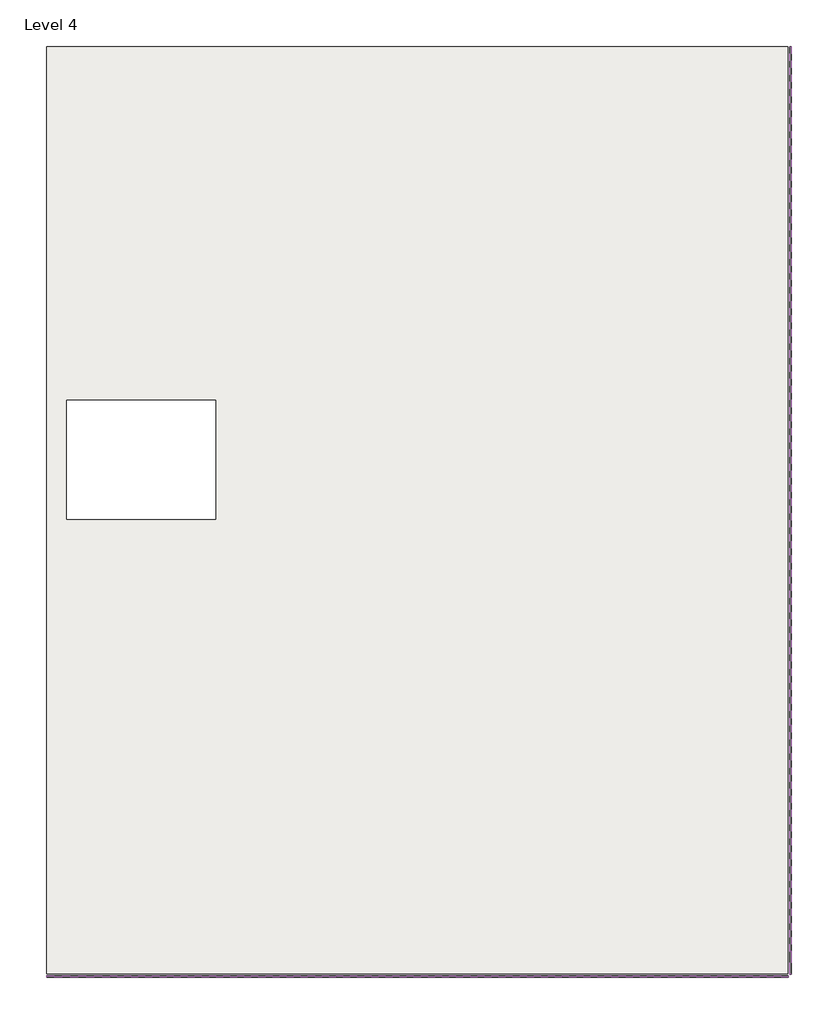
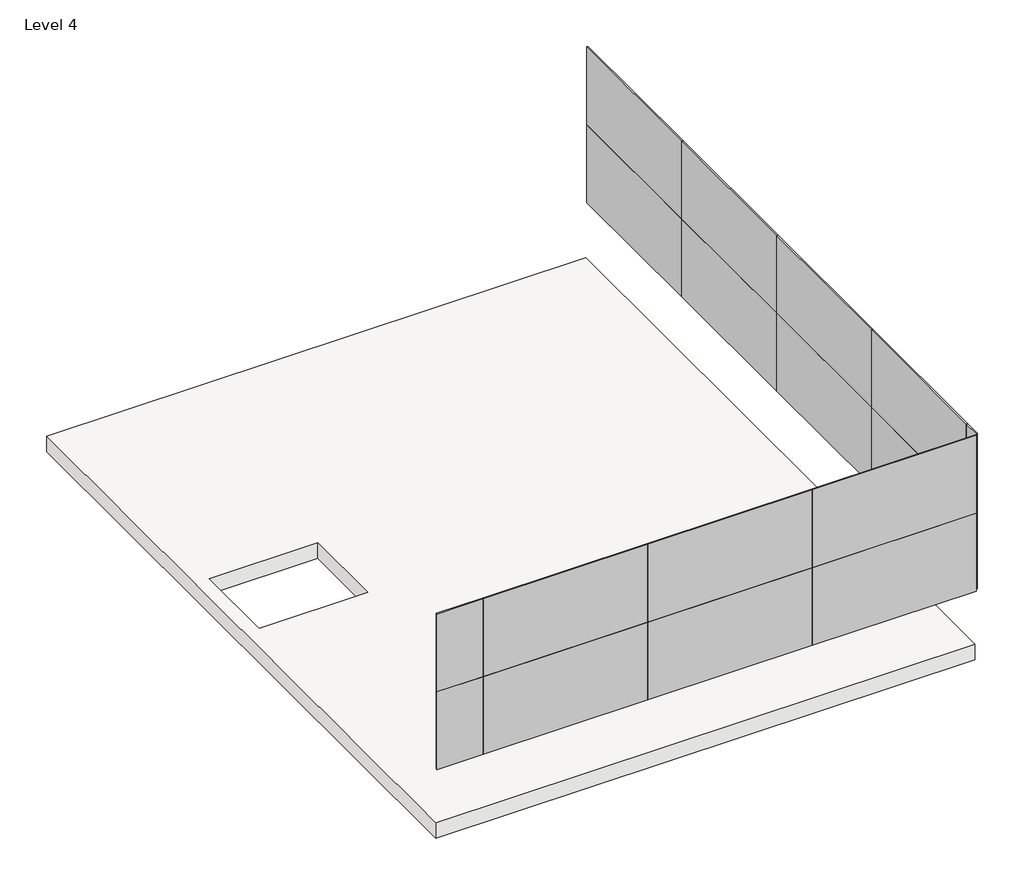
# One storey: 18 plates, 1 slab.
"""IFC4 building model written with IfcOpenShell, lengths in millimetres."""

import ifcopenshell
import ifcopenshell.guid

model = None  # the IFC model being written
_history = None  # IfcOwnerHistory: only IFC2X3 demands one
_inside = {}  # id of a spatial element -> (the spatial element, [elements in it])
_under = {}  # id of a project, library or spatial element -> (it, [spatial elements below it])
_declared = {}  # id of a project -> (the project, [libraries it declares])
_typed = {}  # id of a type object -> (the type object, [elements of that type])
_made_of = {}  # id of a material, layer set ... -> (it, [elements and type objects made of it])


def new_model(schema):
    """Start an empty IFC model of exactly this schema.

    Asked for "IFC4X3", IfcOpenShell would pick the latest addendum, in which some entities
    have other attributes; the version numbers below select the first issue.
    IFC2X3 requires an IfcOwnerHistory on every rooted entity: one is made here for all.
    """
    global model, _history
    if schema == "IFC4X3":
        model = ifcopenshell.file(schema_version=(4, 3, 0, 0))
    else:
        model = ifcopenshell.file(schema=schema)
    _inside.clear()
    _under.clear()
    _declared.clear()
    _typed.clear()
    _made_of.clear()
    _history = None
    if model.schema == "IFC2X3":
        org = make("IfcOrganization", Name="unknown")
        user = make(
            "IfcPersonAndOrganization",
            ThePerson=make("IfcPerson", FamilyName="unknown"),
            TheOrganization=org,
        )
        app = make(
            "IfcApplication",
            ApplicationDeveloper=org,
            Version="unknown",
            ApplicationFullName="unknown",
            ApplicationIdentifier="unknown",
        )
        _history = make(
            "IfcOwnerHistory",
            OwningUser=user,
            OwningApplication=app,
            ChangeAction="ADDED",
            CreationDate=0,
        )
    return model


def make(cls, **values):
    """One entity of the class cls with the attributes given. An attribute that is None is left unset."""
    return model.create_entity(
        cls, **{name: value for name, value in values.items() if value is not None}
    )


def rooted(cls, **values):
    """An entity with a GlobalId (a new one), such as an element, a storey or a relation."""
    return make(cls, GlobalId=ifcopenshell.guid.new(), OwnerHistory=_history, **values)


def si_unit(unit_type, name, prefix=None):
    """IfcSIUnit, for example si_unit("LENGTHUNIT", "METRE", prefix="MILLI")."""
    return make("IfcSIUnit", UnitType=unit_type, Prefix=prefix, Name=name)


def assignment(units):
    """IfcUnitAssignment: the units of a project."""
    return None if units is None else make("IfcUnitAssignment", Units=units)


def point(xyz):
    """IfcCartesianPoint."""
    return None if xyz is None else make("IfcCartesianPoint", Coordinates=xyz)


def direction(xyz):
    """IfcDirection."""
    return None if xyz is None else make("IfcDirection", DirectionRatios=xyz)


def frame(location, z_axis=None, x_axis=None):
    """IfcAxis2Placement3D, a coordinate frame: its origin and axes. An axis left out is left unset."""
    return make(
        "IfcAxis2Placement3D",
        Location=point(location),
        Axis=direction(z_axis),
        RefDirection=direction(x_axis),
    )


def origin():
    """The frame at (0, 0, 0) with its axes left unset."""
    return frame((0.0, 0.0, 0.0))


def origin_with_axes():
    """The frame at (0, 0, 0) with the z axis (0, 0, 1) and the x axis (1, 0, 0) written out."""
    return frame((0.0, 0.0, 0.0), z_axis=(0.0, 0.0, 1.0), x_axis=(1.0, 0.0, 0.0))


def place(relative_to, where):
    """IfcLocalPlacement: puts the frame where relative to a parent placement (None: the world)."""
    return make(
        "IfcLocalPlacement", PlacementRelTo=relative_to, RelativePlacement=where
    )


def context(
    kind, dimensions, precision=None, world=None, true_north=None, identifier=None
):
    """IfcGeometricRepresentationContext, for example the 3D "Model" context."""
    return make(
        "IfcGeometricRepresentationContext",
        ContextIdentifier=identifier,
        ContextType=kind,
        CoordinateSpaceDimension=dimensions,
        Precision=precision,
        WorldCoordinateSystem=world,
        TrueNorth=true_north,
    )


def project(units=None, contexts=None):
    """IfcProject with its units and contexts."""
    return rooted(
        "IfcProject",
        Name="project",
        RepresentationContexts=contexts,
        UnitsInContext=assignment(units),
    )


def spatial(cls, under=None, at=None, **own):
    """A site, building, storey or space (cls), placed at a placement, below another one or the project."""
    s = rooted(cls, ObjectPlacement=at, **own)
    if under is not None:
        _under.setdefault(under.id(), (under, []))[1].append(s)
    return s


def polyline(points):
    """IfcPolyline through the points."""
    return make("IfcPolyline", Points=[point(p) for p in points])


def outline(outer, holes=None, kind="AREA"):
    """IfcArbitraryClosedProfileDef: a profile drawn as a closed curve; with holes, ...WithVoids."""
    if holes is None:
        return make("IfcArbitraryClosedProfileDef", ProfileType=kind, OuterCurve=outer)
    return make(
        "IfcArbitraryProfileDefWithVoids",
        ProfileType=kind,
        OuterCurve=outer,
        InnerCurves=holes,
    )


def extrude(swept, where, along, depth):
    """IfcExtrudedAreaSolid: the profile swept, set in the frame where, extruded along a direction by depth."""
    return make(
        "IfcExtrudedAreaSolid",
        SweptArea=swept,
        Position=where,
        ExtrudedDirection=direction(along),
        Depth=depth,
    )


def shape(context_of_items, identifier, shape_type, items):
    """IfcShapeRepresentation: the items that make up one representation, for example the "Body"."""
    return make(
        "IfcShapeRepresentation",
        ContextOfItems=context_of_items,
        RepresentationIdentifier=identifier,
        RepresentationType=shape_type,
        Items=items,
    )


def source(mapping_origin, context_of_items, identifier, shape_type, items):
    """IfcRepresentationMap: a shape defined once, which mapped items show again and again."""
    return make(
        "IfcRepresentationMap",
        MappingOrigin=mapping_origin,
        MappedRepresentation=shape(context_of_items, identifier, shape_type, items),
    )


def transform(
    local_origin,
    x_axis=None,
    y_axis=None,
    z_axis=None,
    scale=None,
    scale2=None,
    scale3=None,
    uniform=True,
):
    """IfcCartesianTransformationOperator3D, or its non-uniform kind. x_axis, y_axis, z_axis: its Axis1, 2, 3."""
    if uniform:
        return make(
            "IfcCartesianTransformationOperator3D",
            Axis1=direction(x_axis),
            Axis2=direction(y_axis),
            LocalOrigin=point(local_origin),
            Scale=scale,
            Axis3=direction(z_axis),
        )
    return make(
        "IfcCartesianTransformationOperator3DnonUniform",
        Axis1=direction(x_axis),
        Axis2=direction(y_axis),
        LocalOrigin=point(local_origin),
        Scale=scale,
        Axis3=direction(z_axis),
        Scale2=scale2,
        Scale3=scale3,
    )


def mapped(mapping_source, mapping_target):
    """IfcMappedItem: shows the shape of a source again, moved by a transform."""
    return make(
        "IfcMappedItem", MappingSource=mapping_source, MappingTarget=mapping_target
    )


def made_of(thing, what):
    """Note that an element or type object is made of a material, layer set ...; save() writes the relation."""
    if what is not None:
        _made_of.setdefault(what.id(), (what, []))[1].append(thing)
    return thing


def element(
    cls,
    number,
    at=None,
    inside=None,
    cuts=None,
    type_object=None,
    material=None,
    context=None,
    identifier="Body",
    shape_type=None,
    held_by="IfcProductDefinitionShape",
    body=None,
    shapes=None,
    **own,
):
    """One element of the class cls, such as IfcWall. Its Tag is "e" and its number.

    at: its placement. inside: the storey or other place that contains it. cuts: it is an
    opening in that element (IfcRelVoidsElement). A single representation is given by context,
    identifier, shape_type and body (its items); several are given by shapes. held_by: the class
    of the entity that holds the representations. save() writes the other relations.
    """
    e = rooted(cls, Tag="e%d" % number, ObjectPlacement=at, **own)
    if body is not None:
        shapes = [shape(context, identifier, shape_type, body)]
    if shapes is not None:
        e.Representation = make(held_by, Representations=shapes)
    if inside is not None:
        _inside.setdefault(inside.id(), (inside, []))[1].append(e)
    if cuts is not None:
        rooted(
            "IfcRelVoidsElement", RelatingBuildingElement=cuts, RelatedOpeningElement=e
        )
    if type_object is not None:
        _typed.setdefault(type_object.id(), (type_object, []))[1].append(e)
    return made_of(e, material)


def aggregate(whole, parts):
    """IfcRelAggregates: a whole, such as a stair, and the parts it consists of."""
    return rooted("IfcRelAggregates", RelatingObject=whole, RelatedObjects=parts)


def save(model, path):
    """Write the relations noted so far, then the file.

    IfcRelAggregates (storeys below a building ...), IfcRelContainedInSpatialStructure (elements
    in a storey), IfcRelDefinesByType, IfcRelAssociatesMaterial and IfcRelDeclares: one each for
    every whole, place, type object, material and project.
    """
    for whole, parts in _under.values():
        aggregate(whole, parts)
    for where, things in _inside.values():
        rooted(
            "IfcRelContainedInSpatialStructure",
            RelatedElements=things,
            RelatingStructure=where,
        )
    for kind, things in _typed.values():
        rooted("IfcRelDefinesByType", RelatedObjects=things, RelatingType=kind)
    for what, things in _made_of.values():
        rooted("IfcRelAssociatesMaterial", RelatedObjects=things, RelatingMaterial=what)
    for by, libraries in _declared.values():
        rooted("IfcRelDeclares", RelatingContext=by, RelatedDefinitions=libraries)
    model.write(path)


def system_panel_glazed_1e57f9bb(model_context):
    return source(origin(), model_context, "Body", "SweptSolid", [
        extrude(outline(polyline([(1524.0000002, 19.05), (-1524.0000002, 19.05), (-1524.0000002, 44.45), (1524.0000002, 44.45), (1524.0000002, 19.05)])), origin_with_axes(), (0.0, 0.0, 1.0), 1524.0),
    ])


def system_panel_glazed_ccfd9adb(model_context):
    return source(origin(), model_context, "Body", "SweptSolid", [
        extrude(outline(polyline([(427.9999998, 19.05), (-427.9999998, 19.05), (-427.9999998, 44.45), (427.9999998, 44.45), (427.9999998, 19.05)])), origin_with_axes(), (0.0, 0.0, 1.0), 1524.0),
    ])


def system_panel_glazed_88f24eba(model_context):
    return source(origin(), model_context, "Body", "SweptSolid", [
        extrude(outline(polyline([(153.9999998, 19.05), (-153.9999998, 19.05), (-153.9999998, 44.45), (153.9999998, 44.45), (153.9999998, 19.05)])), origin_with_axes(), (0.0, 0.0, 1.0), 1524.0),
    ])


model = new_model("IFC4")

# Units and contexts
model_context = context("Model", 3, world=origin())
ifc_project = project(units=[si_unit("LENGTHUNIT", "METRE", prefix="MILLI")], contexts=[model_context])

# Site, building, storey
site = spatial("IfcSite", under=ifc_project)
building = spatial("IfcBuilding", under=site)
storey = spatial("IfcBuildingStorey", under=building, Name="Level 4", Elevation=9600.0)

# Plates
placement = place(None, origin())
system_panel_glazed_shape = system_panel_glazed_1e57f9bb(model_context)
element("IfcPlate", 1, ObjectType="System Panel : Glazed", at=placement, inside=storey, context=model_context, shape_type="MappedRepresentation", body=[
    mapped(system_panel_glazed_shape, transform((2137.6340362, 1399.6955828, 10668.0), x_axis=(-1.0, 0.0, 0.0), y_axis=(0.0, -1.0, 0.0), z_axis=(0.0, 0.0, 1.0))),
])
element("IfcPlate", 2, ObjectType="System Panel : Glazed", at=placement, inside=storey, context=model_context, shape_type="MappedRepresentation", body=[
    mapped(system_panel_glazed_shape, transform((-910.3659639, 1399.6955828, 10668.0), x_axis=(-1.0, 0.0, 0.0), y_axis=(0.0, -1.0, 0.0), z_axis=(0.0, 0.0, 1.0))),
])
element("IfcPlate", 3, ObjectType="System Panel : Glazed", at=placement, inside=storey, context=model_context, shape_type="MappedRepresentation", body=[
    mapped(system_panel_glazed_shape, transform((-3958.3659639, 1399.6955828, 10668.0), x_axis=(-1.0, 0.0, 0.0), y_axis=(0.0, -1.0, 0.0), z_axis=(0.0, 0.0, 1.0))),
])
element("IfcPlate", 4, ObjectType="System Panel : Glazed", at=placement, inside=storey, context=model_context, shape_type="MappedRepresentation", body=[
    mapped(system_panel_glazed_shape, transform((2137.6340362, 1399.6955828, 12192.0), x_axis=(-1.0, 0.0, 0.0), y_axis=(0.0, -1.0, 0.0), z_axis=(0.0, 0.0, 1.0))),
])
element("IfcPlate", 5, ObjectType="System Panel : Glazed", at=placement, inside=storey, context=model_context, shape_type="MappedRepresentation", body=[
    mapped(system_panel_glazed_shape, transform((-910.3659639, 1399.6955828, 12192.0), x_axis=(-1.0, 0.0, 0.0), y_axis=(0.0, -1.0, 0.0), z_axis=(0.0, 0.0, 1.0))),
])
element("IfcPlate", 6, ObjectType="System Panel : Glazed", at=placement, inside=storey, context=model_context, shape_type="MappedRepresentation", body=[
    mapped(system_panel_glazed_shape, transform((-3958.3659639, 1399.6955828, 12192.0), x_axis=(-1.0, 0.0, 0.0), y_axis=(0.0, -1.0, 0.0), z_axis=(0.0, 0.0, 1.0))),
])
element("IfcPlate", 7, ObjectType="System Panel : Glazed", at=placement, inside=storey, context=model_context, shape_type="MappedRepresentation", body=[
    mapped(system_panel_glazed_shape, transform((3661.6340364, 12375.6955827, 10668.0), x_axis=(0.0, -1.0, 0.0), y_axis=(1.0, 0.0, 0.0), z_axis=(0.0, 0.0, 1.0))),
])
element("IfcPlate", 8, ObjectType="System Panel : Glazed", at=placement, inside=storey, context=model_context, shape_type="MappedRepresentation", body=[
    mapped(system_panel_glazed_shape, transform((3661.6340364, 9327.6955825, 10668.0), x_axis=(0.0, -1.0, 0.0), y_axis=(1.0, 0.0, 0.0), z_axis=(0.0, 0.0, 1.0))),
])
element("IfcPlate", 9, ObjectType="System Panel : Glazed", at=placement, inside=storey, context=model_context, shape_type="MappedRepresentation", body=[
    mapped(system_panel_glazed_shape, transform((3661.6340364, 6279.6955825, 10668.0), x_axis=(0.0, -1.0, 0.0), y_axis=(1.0, 0.0, 0.0), z_axis=(0.0, 0.0, 1.0))),
])
element("IfcPlate", 10, ObjectType="System Panel : Glazed", at=placement, inside=storey, context=model_context, shape_type="MappedRepresentation", body=[
    mapped(system_panel_glazed_shape, transform((3661.6340364, 3231.6955825, 10668.0), x_axis=(0.0, -1.0, 0.0), y_axis=(1.0, 0.0, 0.0), z_axis=(0.0, 0.0, 1.0))),
])
element("IfcPlate", 11, ObjectType="System Panel : Glazed", at=placement, inside=storey, context=model_context, shape_type="MappedRepresentation", body=[
    mapped(system_panel_glazed_shape, transform((3661.6340364, 12375.6955827, 12192.0), x_axis=(0.0, -1.0, 0.0), y_axis=(1.0, 0.0, 0.0), z_axis=(0.0, 0.0, 1.0))),
])
element("IfcPlate", 12, ObjectType="System Panel : Glazed", at=placement, inside=storey, context=model_context, shape_type="MappedRepresentation", body=[
    mapped(system_panel_glazed_shape, transform((3661.6340364, 9327.6955825, 12192.0), x_axis=(0.0, -1.0, 0.0), y_axis=(1.0, 0.0, 0.0), z_axis=(0.0, 0.0, 1.0))),
])
element("IfcPlate", 13, ObjectType="System Panel : Glazed", at=placement, inside=storey, context=model_context, shape_type="MappedRepresentation", body=[
    mapped(system_panel_glazed_shape, transform((3661.6340364, 6279.6955825, 12192.0), x_axis=(0.0, -1.0, 0.0), y_axis=(1.0, 0.0, 0.0), z_axis=(0.0, 0.0, 1.0))),
])
element("IfcPlate", 14, ObjectType="System Panel : Glazed", at=placement, inside=storey, context=model_context, shape_type="MappedRepresentation", body=[
    mapped(system_panel_glazed_shape, transform((3661.6340364, 3231.6955825, 12192.0), x_axis=(0.0, -1.0, 0.0), y_axis=(1.0, 0.0, 0.0), z_axis=(0.0, 0.0, 1.0))),
])
system_panel_glazed_2_shape = system_panel_glazed_ccfd9adb(model_context)
element("IfcPlate", 15, ObjectType="System Panel : Glazed", at=placement, inside=storey, context=model_context, shape_type="MappedRepresentation", body=[
    mapped(system_panel_glazed_2_shape, transform((-5910.3659638, 1399.6955828, 10668.0), x_axis=(-1.0, 0.0, 0.0), y_axis=(0.0, -1.0, 0.0), z_axis=(0.0, 0.0, 1.0))),
])
element("IfcPlate", 16, ObjectType="System Panel : Glazed", at=placement, inside=storey, context=model_context, shape_type="MappedRepresentation", body=[
    mapped(system_panel_glazed_2_shape, transform((-5910.3659638, 1399.6955828, 12192.0), x_axis=(-1.0, 0.0, 0.0), y_axis=(0.0, -1.0, 0.0), z_axis=(0.0, 0.0, 1.0))),
])
system_panel_glazed_3_shape = system_panel_glazed_88f24eba(model_context)
element("IfcPlate", 17, ObjectType="System Panel : Glazed", at=placement, inside=storey, context=model_context, shape_type="MappedRepresentation", body=[
    mapped(system_panel_glazed_3_shape, transform((3661.6340364, 1553.6955827, 10668.0), x_axis=(0.0, -1.0, 0.0), y_axis=(1.0, 0.0, 0.0), z_axis=(0.0, 0.0, 1.0))),
])
element("IfcPlate", 18, ObjectType="System Panel : Glazed", at=placement, inside=storey, context=model_context, shape_type="MappedRepresentation", body=[
    mapped(system_panel_glazed_3_shape, transform((3661.6340364, 1553.6955827, 12192.0), x_axis=(0.0, -1.0, 0.0), y_axis=(1.0, 0.0, 0.0), z_axis=(0.0, 0.0, 1.0))),
])

# Slab
element("IfcSlab", 19, ObjectType="Generic - 12\"", at=placement, inside=storey, context=model_context, shape_type="SweptSolid", body=[
    extrude(outline(polyline([(-6335.3659636, 1402.6955828), (-6335.3659636, 13896.6955828), (3658.6340364, 13896.6955828), (3658.6340364, 1402.6955828), (-6335.3659636, 1402.6955828)]), holes=[polyline([(-4059.8993101, 7527.9023719), (-4059.8993101, 9133.9023719), (-6065.8993101, 9133.9023719), (-6065.8993101, 7527.9023719), (-4059.8993101, 7527.9023719)])]), frame((0.0, 0.0, 9295.2), z_axis=(0.0, 0.0, 1.0), x_axis=(1.0, 0.0, 0.0)), (0.0, 0.0, 1.0), 304.8),
])

save(model, "model.ifc")

# Revit data of these elements
# Type "System Panel : Glazed"
#   Construction Type Id = "GSP4R"
#   Analytic Construction = "1/8 in Pilkington single glazing"
#   Visual Light Transmittance = 0.9
#   Solar Heat Gain Coefficient = 0.86
#   Heat Transfer Coefficient (U) = 6.7069 W/(m²·K)
# Type "Generic - 12\""
#   Assembly Code = "B1010"
#   Function = 0
#   Layers, outside or top first: 0.3048 m no material (function 1)
# Elements 1, 2, 3, 4, 5, 6, 7, 8, 9, 10, 11, 12, 13, 14, 15, 16, 17, 18 (IfcPlate, "System Panel : Glazed")
#   Phase Created = New Construction
#   Materials on its faces: "Glass"
# Element 19 (IfcSlab, "Generic - 12\"")
#   built-in parameter 1001955 = -1.5708 (stored number, unit not read)
#   Height Offset From Level = 0.00 m
#   Phase Created = New Construction
#   Materials on its faces: "Default Floor"
# Materials
#   "Glass": class "Glass", colour RGB 0 128 192, transparency 0.75, Description = "Soda Lime Glass", Cost = 0
#   "Default Floor": class "Miscellaneous", colour RGB 128 128 128, transparency 0, Cost = 0
